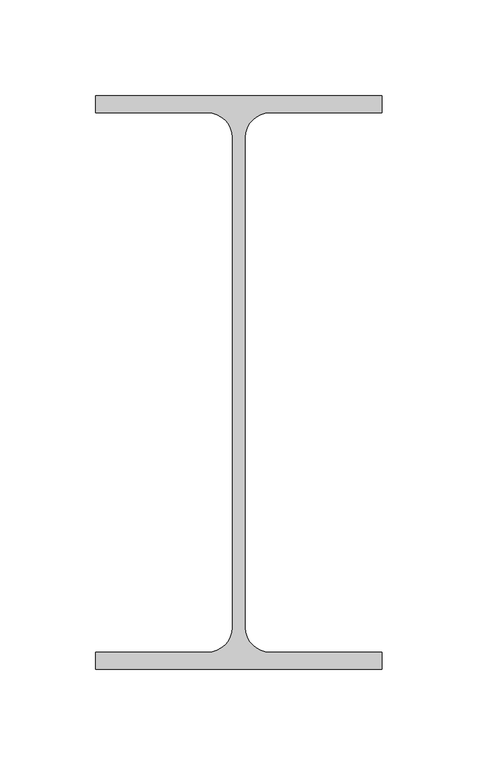
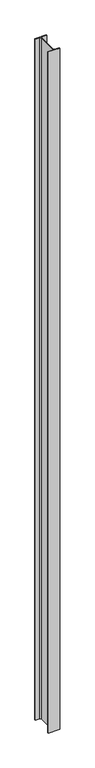
"""IFC4 building model written with IfcOpenShell, lengths in millimetres: column geometry, Steel Column_H_KS : H_SC_AR_S01_H-300x150x6.5x9_SSC1."""

from ifc_helpers import new_model, si_unit, point, frame, frame_2d, origin, place, context, project, spatial, polyline, circle_curve, trimmed, segment, composite_curve, outline, extrude, source, transform, mapped, element, save


def column_97af4cd3(model_context):
    return source(origin(), model_context, "Body", "SweptSolid", [
        extrude(outline(composite_curve([segment(polyline([(75.0, 150.0), (75.0, 141.0), (16.25, 141.0)]), True, "CONTINUOUS"), segment(trimmed(circle_curve(frame_2d((16.25, 128.0)), 13.0), [point((16.25, 141.0))], [point((3.25, 128.0))], True, "CARTESIAN"), True, "CONTINUOUS"), segment(polyline([(3.25, 128.0), (3.25, -128.0)]), True, "CONTINUOUS"), segment(trimmed(circle_curve(frame_2d((16.25, -128.0)), 13.0), [point((3.25, -128.0))], [point((16.25, -141.0))], True, "CARTESIAN"), True, "CONTINUOUS"), segment(polyline([(16.25, -141.0), (75.0, -141.0), (75.0, -150.0), (-75.0, -150.0), (-75.0, -141.0), (-16.25, -141.0)]), True, "CONTINUOUS"), segment(trimmed(circle_curve(frame_2d((-16.25, -128.0)), 13.0), [point((-16.25, -141.0))], [point((-3.25, -128.0))], True, "CARTESIAN"), True, "CONTINUOUS"), segment(polyline([(-3.25, -128.0), (-3.25, 128.0)]), True, "CONTINUOUS"), segment(trimmed(circle_curve(frame_2d((-16.25, 128.0)), 13.0), [point((-3.25, 128.0))], [point((-16.25, 141.0))], True, "CARTESIAN"), True, "CONTINUOUS"), segment(polyline([(-16.25, 141.0), (-75.0, 141.0), (-75.0, 150.0), (75.0, 150.0)]), True, "CONTINUOUS")], self_intersect=False)), frame((0.0, 0.0, 249.9618634), z_axis=(0.0, 0.0, 1.0), x_axis=(1.0, 0.0, 0.0)), (0.0, 0.0, 1.0), 9350.0),
    ])


if __name__ == "__main__":
    model = new_model("IFC4")
    model_context = context("Model", 3, world=origin())
    ifc_project = project(units=[si_unit("LENGTHUNIT", "METRE", prefix="MILLI")], contexts=[model_context])
    site = spatial("IfcSite", under=ifc_project)
    building = spatial("IfcBuilding", under=site)
    placement = place(None, origin())
    column_shape = column_97af4cd3(model_context)
    element("IfcColumn", 1, ObjectType="Steel Column_H_KS : H_SC_AR_S01_H-300x150x6.5x9_SSC1", at=placement, inside=building, context=model_context, shape_type="MappedRepresentation", body=[
        mapped(column_shape, transform((0.0, 0.0, 0.0), x_axis=(1.0, 0.0, 0.0), y_axis=(0.0, 1.0, 0.0), z_axis=(0.0, 0.0, 1.0))),
    ])
    save(model, "model.ifc")

# Revit data of these elements
# Type "Steel Column_H_KS : H_SC_AR_S01_H-300x150x6.5x9_SSC1"
#   Type Comments = "MAIN"
#   Type Mark = "SSC1"
#   H_SectionID = "H-300x150x6.5x9"
#   H_Ratio for Additional Steel Plate = 0.2
#   Width = 15.0 cm
#   Web Thickness = 0.65 cm
#   Web Fillet = 1.3 cm
#   Warping Constant = 107174.4 cm⁶
#   Torsional Moment of Inertia = 9.95386 cm⁴
#   Section Area = 46.78 cm²
#   Plastic Modulus weak axis = 105.0 cm³
#   Plastic Modulus strong axis = 542.0 cm³
#   Perimeter = 1.165 m²/m
#   Nominal Weight = 36.70 kgf/m
#   Moment of Inertia weak axis = 508.00 cm⁴
#   Moment of Inertia strong axis = 7210.00 cm⁴
#   Height = 30.0 cm
#   Flange Thickness = 0.9 cm
#   Elastic Modulus weak axis = 67.7 cm³
#   Elastic Modulus strong axis = 481.0 cm³
#   Centroid Vertical = 15.0 cm
#   Centroid Horizontal = 7.5 cm
#   Structural Material [instance default] = Steel, 45-345
#   Section Name Key = ""
#   Bolt Spacing = 0
#   Assembly Code = ""
# Element 1 (IfcColumn, "Steel Column_H_KS : H_SC_AR_S01_H-300x150x6.5x9_SSC1")
#   Materials on its faces: "Steel, 45-345"
# Materials
#   "Steel, 45-345": class "Metal", colour RGB 189 187 185, transparency 0, Description = "Steel 345 MPa", Cost = 0
